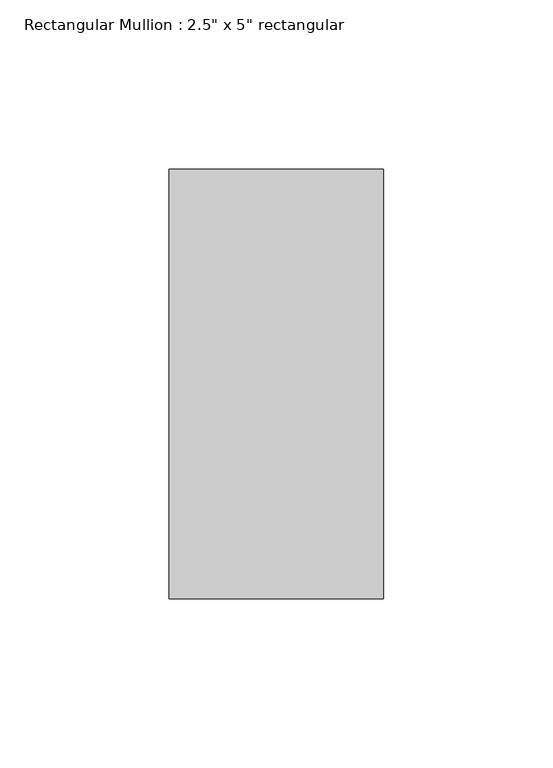
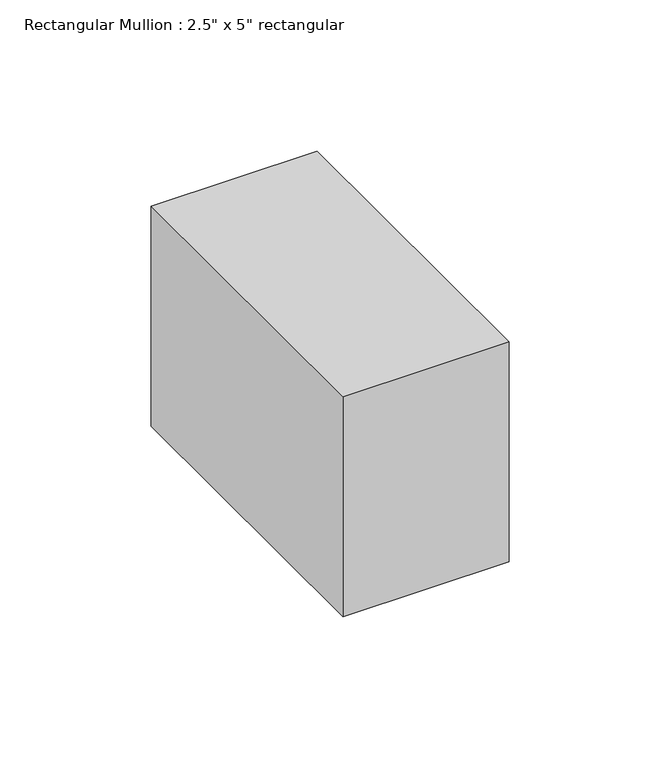
"""IFC4 building model written with IfcOpenShell, lengths in millimetres: member geometry."""

from ifc_helpers import new_model, si_unit, frame, origin, place, context, project, spatial, polyline, outline, extrude, source, transform, mapped, element, save


def member_7712ce12(model_context):
    return source(origin(), model_context, "Body", "SweptSolid", [
        extrude(outline(polyline([(0.0, 63.5), (0.0, -63.5), (-63.5, -63.5), (-63.5, 63.5), (0.0, 63.5)])), frame((0.0, 0.0, -88.9), z_axis=(0.0, 0.0, 1.0), x_axis=(1.0, 0.0, 0.0)), (0.0, 0.0, 1.0), 88.9),
    ])


if __name__ == "__main__":
    model = new_model("IFC4")
    model_context = context("Model", 3, world=origin())
    ifc_project = project(units=[si_unit("LENGTHUNIT", "METRE", prefix="MILLI")], contexts=[model_context])
    site = spatial("IfcSite", under=ifc_project)
    building = spatial("IfcBuilding", under=site)
    placement = place(None, origin())
    member_shape = member_7712ce12(model_context)
    element("IfcMember", 1, ObjectType="Rectangular Mullion : 2.5\" x 5\" rectangular", at=placement, inside=building, context=model_context, shape_type="MappedRepresentation", body=[
        mapped(member_shape, transform((0.0, 0.0, 0.0), x_axis=(1.0, 0.0, 0.0), y_axis=(0.0, 1.0, 0.0), z_axis=(0.0, 0.0, 1.0))),
    ])
    save(model, "model.ifc")

# Revit data of these elements
# Type "Rectangular Mullion : 2.5\" x 5\" rectangular"
#   built-in parameter 1007304 = 0.416667 (stored number, unit not read)
#   built-in parameter 1007301 = 0.104167 (stored number, unit not read)
#   built-in parameter 1007300 = 0.104167 (stored number, unit not read)
# Element 1 (IfcMember, "Rectangular Mullion : 2.5\" x 5\" rectangular")
#   Materials on its faces: "Metal - Aluminum"
# Materials
#   "Metal - Aluminum": class "Metal", colour RGB 140 140 140, transparency 0
